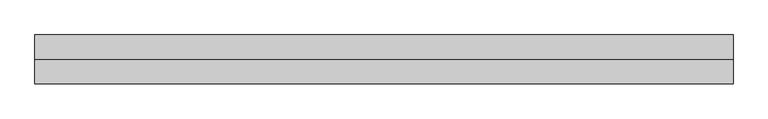
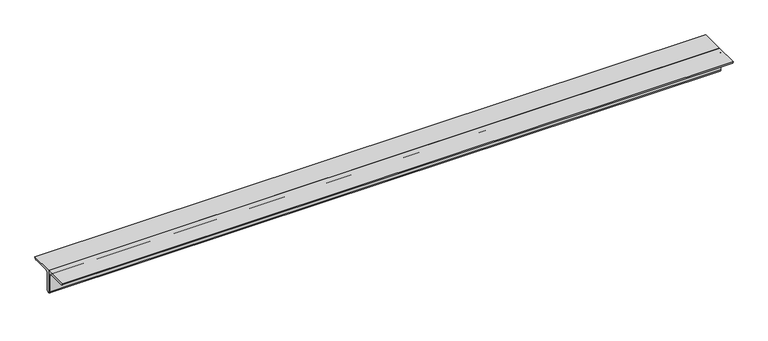
"""IFC4 building model written with IfcOpenShell, lengths in millimetres: member geometry, 0123_Steel Framing_2Ls-KSD3502 : H_SB_AR_S03_2Ls-130x130x12_HBR1."""

from ifc_helpers import new_model, si_unit, point, frame, frame_2d, origin, place, context, project, spatial, polyline, circle_curve, trimmed, segment, composite_curve, outline, extrude, source, transform, mapped, element, save


def member_48b3af6f(model_context):
    return source(origin(), model_context, "Body", "SweptSolid", [
        extrude(outline(composite_curve([segment(polyline([(0.0, 36.4), (130.0, 36.4)]), True, "CONTINUOUS"), segment(trimmed(circle_curve(frame_2d((118.0, 36.4)), 12.0), [point((130.0, 36.4))], [point((118.0, 24.4))], False, "CARTESIAN"), True, "CONTINUOUS"), segment(polyline([(118.0, 24.4), (24.0, 24.4)]), True, "CONTINUOUS"), segment(trimmed(circle_curve(frame_2d((24.0, 12.4)), 12.0), [point((24.0, 24.4))], [point((12.0, 12.4))], True, "CARTESIAN"), True, "CONTINUOUS"), segment(polyline([(12.0, 12.4), (12.0, -81.6)]), True, "CONTINUOUS"), segment(trimmed(circle_curve(frame_2d((0.0, -81.6)), 12.0), [point((12.0, -81.6))], [point((0.0, -93.6))], False, "CARTESIAN"), True, "CONTINUOUS"), segment(polyline([(0.0, -93.6), (0.0, 36.4)]), True, "CONTINUOUS")], self_intersect=False)), frame((-1830.7666695, 0.0, 0.0), z_axis=(1.0, 0.0, 0.0), x_axis=(0.0, 1.0, 0.0)), (0.0, 0.0, 1.0), 3701.6272171),
        extrude(outline(composite_curve([segment(polyline([(0.0, 36.4), (0.0, -93.6)]), True, "CONTINUOUS"), segment(trimmed(circle_curve(frame_2d((0.0, -81.6)), 12.0), [point((0.0, -93.6))], [point((-12.0, -81.6))], False, "CARTESIAN"), True, "CONTINUOUS"), segment(polyline([(-12.0, -81.6), (-12.0, 12.4)]), True, "CONTINUOUS"), segment(trimmed(circle_curve(frame_2d((-24.0, 12.4)), 12.0), [point((-12.0, 12.4))], [point((-24.0, 24.4))], True, "CARTESIAN"), True, "CONTINUOUS"), segment(polyline([(-24.0, 24.4), (-118.0, 24.4)]), True, "CONTINUOUS"), segment(trimmed(circle_curve(frame_2d((-118.0, 36.4)), 12.0), [point((-118.0, 24.4))], [point((-130.0, 36.4))], False, "CARTESIAN"), True, "CONTINUOUS"), segment(polyline([(-130.0, 36.4), (0.0, 36.4)]), True, "CONTINUOUS")], self_intersect=False)), frame((-1830.7666695, 0.0, 0.0), z_axis=(1.0, 0.0, 0.0), x_axis=(0.0, 1.0, 0.0)), (0.0, 0.0, 1.0), 3701.6272171),
    ])


if __name__ == "__main__":
    model = new_model("IFC4")
    model_context = context("Model", 3, world=origin())
    ifc_project = project(units=[si_unit("LENGTHUNIT", "METRE", prefix="MILLI")], contexts=[model_context])
    site = spatial("IfcSite", under=ifc_project)
    building = spatial("IfcBuilding", under=site)
    placement = place(None, origin())
    member_shape = member_48b3af6f(model_context)
    element("IfcMember", 1, ObjectType="0123_Steel Framing_2Ls-KSD3502 : H_SB_AR_S03_2Ls-130x130x12_HBR1", at=placement, inside=building, context=model_context, shape_type="MappedRepresentation", body=[
        mapped(member_shape, transform((0.0, 0.0, 0.0), x_axis=(1.0, 0.0, 0.0), y_axis=(0.0, 1.0, 0.0), z_axis=(0.0, 0.0, 1.0))),
    ])
    save(model, "model.ifc")

# Revit data of these elements
# Type "0123_Steel Framing_2Ls-KSD3502 : H_SB_AR_S03_2Ls-130x130x12_HBR1"
#   Type Mark = "HBR1"
#   Assembly Code = "B10"
#   Legs = "SLBB"
#   W = 8.97
#   Perimeter = 1.04 m²/m
#   Nominal Weight = 46.80 kgf/m
#   Length [instance default] = 1000 mm
#   Space = 0 mm
#   b = 130 mm
#   d = 130 mm
#   t = 12 mm
#   y = 36.4 mm
#   A = 0.005952 m²
#   Structural Material [instance default] = Steel ASTM A36
# Element 1 (IfcMember, "0123_Steel Framing_2Ls-KSD3502 : H_SB_AR_S03_2Ls-130x130x12_HBR1")
#   Materials on its faces: "Steel ASTM A36"
# Materials
#   "Steel ASTM A36": class "Metal", colour RGB 199 199 199, transparency 0, Description = "Structural steel, ASTM A36 Grade B, mill finish", Cost = 0
